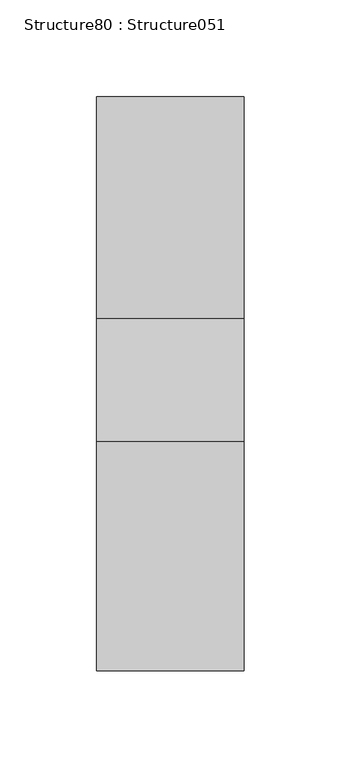
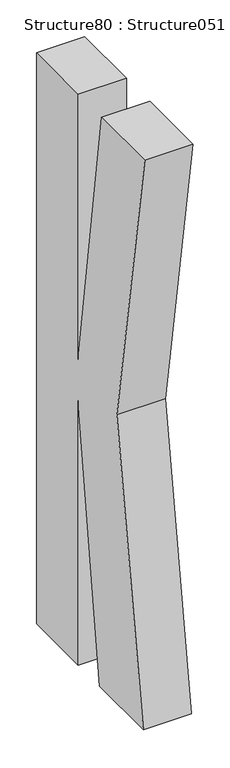
"""IFC4 building model written with IfcOpenShell, lengths in millimetres: proxy geometry, Structure80 : Structure051."""

import ifcopenshell
import ifcopenshell.guid

model = None  # the IFC model being written
_history = None  # IfcOwnerHistory: only IFC2X3 demands one
_inside = {}  # id of a spatial element -> (the spatial element, [elements in it])
_under = {}  # id of a project, library or spatial element -> (it, [spatial elements below it])
_declared = {}  # id of a project -> (the project, [libraries it declares])
_typed = {}  # id of a type object -> (the type object, [elements of that type])
_made_of = {}  # id of a material, layer set ... -> (it, [elements and type objects made of it])


def new_model(schema):
    """Start an empty IFC model of exactly this schema.

    Asked for "IFC4X3", IfcOpenShell would pick the latest addendum, in which some entities
    have other attributes; the version numbers below select the first issue.
    IFC2X3 requires an IfcOwnerHistory on every rooted entity: one is made here for all.
    """
    global model, _history
    if schema == "IFC4X3":
        model = ifcopenshell.file(schema_version=(4, 3, 0, 0))
    else:
        model = ifcopenshell.file(schema=schema)
    _inside.clear()
    _under.clear()
    _declared.clear()
    _typed.clear()
    _made_of.clear()
    _history = None
    if model.schema == "IFC2X3":
        org = make("IfcOrganization", Name="unknown")
        user = make(
            "IfcPersonAndOrganization",
            ThePerson=make("IfcPerson", FamilyName="unknown"),
            TheOrganization=org,
        )
        app = make(
            "IfcApplication",
            ApplicationDeveloper=org,
            Version="unknown",
            ApplicationFullName="unknown",
            ApplicationIdentifier="unknown",
        )
        _history = make(
            "IfcOwnerHistory",
            OwningUser=user,
            OwningApplication=app,
            ChangeAction="ADDED",
            CreationDate=0,
        )
    return model


def make(cls, **values):
    """One entity of the class cls with the attributes given. An attribute that is None is left unset."""
    return model.create_entity(
        cls, **{name: value for name, value in values.items() if value is not None}
    )


def rooted(cls, **values):
    """An entity with a GlobalId (a new one), such as an element, a storey or a relation."""
    return make(cls, GlobalId=ifcopenshell.guid.new(), OwnerHistory=_history, **values)


def si_unit(unit_type, name, prefix=None):
    """IfcSIUnit, for example si_unit("LENGTHUNIT", "METRE", prefix="MILLI")."""
    return make("IfcSIUnit", UnitType=unit_type, Prefix=prefix, Name=name)


def assignment(units):
    """IfcUnitAssignment: the units of a project."""
    return None if units is None else make("IfcUnitAssignment", Units=units)


def point(xyz):
    """IfcCartesianPoint."""
    return None if xyz is None else make("IfcCartesianPoint", Coordinates=xyz)


def direction(xyz):
    """IfcDirection."""
    return None if xyz is None else make("IfcDirection", DirectionRatios=xyz)


def frame(location, z_axis=None, x_axis=None):
    """IfcAxis2Placement3D, a coordinate frame: its origin and axes. An axis left out is left unset."""
    return make(
        "IfcAxis2Placement3D",
        Location=point(location),
        Axis=direction(z_axis),
        RefDirection=direction(x_axis),
    )


def origin():
    """The frame at (0, 0, 0) with its axes left unset."""
    return frame((0.0, 0.0, 0.0))


def place(relative_to, where):
    """IfcLocalPlacement: puts the frame where relative to a parent placement (None: the world)."""
    return make(
        "IfcLocalPlacement", PlacementRelTo=relative_to, RelativePlacement=where
    )


def context(
    kind, dimensions, precision=None, world=None, true_north=None, identifier=None
):
    """IfcGeometricRepresentationContext, for example the 3D "Model" context."""
    return make(
        "IfcGeometricRepresentationContext",
        ContextIdentifier=identifier,
        ContextType=kind,
        CoordinateSpaceDimension=dimensions,
        Precision=precision,
        WorldCoordinateSystem=world,
        TrueNorth=true_north,
    )


def project(units=None, contexts=None):
    """IfcProject with its units and contexts."""
    return rooted(
        "IfcProject",
        Name="project",
        RepresentationContexts=contexts,
        UnitsInContext=assignment(units),
    )


def spatial(cls, under=None, at=None, **own):
    """A site, building, storey or space (cls), placed at a placement, below another one or the project."""
    s = rooted(cls, ObjectPlacement=at, **own)
    if under is not None:
        _under.setdefault(under.id(), (under, []))[1].append(s)
    return s


def polyline(points):
    """IfcPolyline through the points."""
    return make("IfcPolyline", Points=[point(p) for p in points])


def outline(outer, holes=None, kind="AREA"):
    """IfcArbitraryClosedProfileDef: a profile drawn as a closed curve; with holes, ...WithVoids."""
    if holes is None:
        return make("IfcArbitraryClosedProfileDef", ProfileType=kind, OuterCurve=outer)
    return make(
        "IfcArbitraryProfileDefWithVoids",
        ProfileType=kind,
        OuterCurve=outer,
        InnerCurves=holes,
    )


def extrude(swept, where, along, depth):
    """IfcExtrudedAreaSolid: the profile swept, set in the frame where, extruded along a direction by depth."""
    return make(
        "IfcExtrudedAreaSolid",
        SweptArea=swept,
        Position=where,
        ExtrudedDirection=direction(along),
        Depth=depth,
    )


def shape(context_of_items, identifier, shape_type, items):
    """IfcShapeRepresentation: the items that make up one representation, for example the "Body"."""
    return make(
        "IfcShapeRepresentation",
        ContextOfItems=context_of_items,
        RepresentationIdentifier=identifier,
        RepresentationType=shape_type,
        Items=items,
    )


def source(mapping_origin, context_of_items, identifier, shape_type, items):
    """IfcRepresentationMap: a shape defined once, which mapped items show again and again."""
    return make(
        "IfcRepresentationMap",
        MappingOrigin=mapping_origin,
        MappedRepresentation=shape(context_of_items, identifier, shape_type, items),
    )


def transform(
    local_origin,
    x_axis=None,
    y_axis=None,
    z_axis=None,
    scale=None,
    scale2=None,
    scale3=None,
    uniform=True,
):
    """IfcCartesianTransformationOperator3D, or its non-uniform kind. x_axis, y_axis, z_axis: its Axis1, 2, 3."""
    if uniform:
        return make(
            "IfcCartesianTransformationOperator3D",
            Axis1=direction(x_axis),
            Axis2=direction(y_axis),
            LocalOrigin=point(local_origin),
            Scale=scale,
            Axis3=direction(z_axis),
        )
    return make(
        "IfcCartesianTransformationOperator3DnonUniform",
        Axis1=direction(x_axis),
        Axis2=direction(y_axis),
        LocalOrigin=point(local_origin),
        Scale=scale,
        Axis3=direction(z_axis),
        Scale2=scale2,
        Scale3=scale3,
    )


def mapped(mapping_source, mapping_target):
    """IfcMappedItem: shows the shape of a source again, moved by a transform."""
    return make(
        "IfcMappedItem", MappingSource=mapping_source, MappingTarget=mapping_target
    )


def made_of(thing, what):
    """Note that an element or type object is made of a material, layer set ...; save() writes the relation."""
    if what is not None:
        _made_of.setdefault(what.id(), (what, []))[1].append(thing)
    return thing


def element(
    cls,
    number,
    at=None,
    inside=None,
    cuts=None,
    type_object=None,
    material=None,
    context=None,
    identifier="Body",
    shape_type=None,
    held_by="IfcProductDefinitionShape",
    body=None,
    shapes=None,
    **own,
):
    """One element of the class cls, such as IfcWall. Its Tag is "e" and its number.

    at: its placement. inside: the storey or other place that contains it. cuts: it is an
    opening in that element (IfcRelVoidsElement). A single representation is given by context,
    identifier, shape_type and body (its items); several are given by shapes. held_by: the class
    of the entity that holds the representations. save() writes the other relations.
    """
    e = rooted(cls, Tag="e%d" % number, ObjectPlacement=at, **own)
    if body is not None:
        shapes = [shape(context, identifier, shape_type, body)]
    if shapes is not None:
        e.Representation = make(held_by, Representations=shapes)
    if inside is not None:
        _inside.setdefault(inside.id(), (inside, []))[1].append(e)
    if cuts is not None:
        rooted(
            "IfcRelVoidsElement", RelatingBuildingElement=cuts, RelatedOpeningElement=e
        )
    if type_object is not None:
        _typed.setdefault(type_object.id(), (type_object, []))[1].append(e)
    return made_of(e, material)


def aggregate(whole, parts):
    """IfcRelAggregates: a whole, such as a stair, and the parts it consists of."""
    return rooted("IfcRelAggregates", RelatingObject=whole, RelatedObjects=parts)


def save(model, path):
    """Write the relations noted so far, then the file.

    IfcRelAggregates (storeys below a building ...), IfcRelContainedInSpatialStructure (elements
    in a storey), IfcRelDefinesByType, IfcRelAssociatesMaterial and IfcRelDeclares: one each for
    every whole, place, type object, material and project.
    """
    for whole, parts in _under.values():
        aggregate(whole, parts)
    for where, things in _inside.values():
        rooted(
            "IfcRelContainedInSpatialStructure",
            RelatedElements=things,
            RelatingStructure=where,
        )
    for kind, things in _typed.values():
        rooted("IfcRelDefinesByType", RelatedObjects=things, RelatingType=kind)
    for what, things in _made_of.values():
        rooted("IfcRelAssociatesMaterial", RelatedObjects=things, RelatingMaterial=what)
    for by, libraries in _declared.values():
        rooted("IfcRelDeclares", RelatingContext=by, RelatedDefinitions=libraries)
    model.write(path)


def structure80_structure051_452593a8(model_context):
    return source(origin(), model_context, "Body", "SweptSolid", [
        extrude(outline(polyline([(283220.0273561, 3528.5825142), (283292.1031415, 4009.9589531), (283215.9425682, 4480.4419946), (283334.2458585, 4480.4419946), (283398.1520682, 4038.5077532), (283398.1520682, 4480.4419946), (283512.3963918, 4480.4419946), (283512.3963918, 3528.5825142), (283398.1520682, 3528.5825142), (283398.1520682, 3969.1658661), (283339.6865742, 3528.5825142), (283220.0273561, 3528.5825142)])), frame((-59031.6926606, 0.0, 0.0), z_axis=(1.0, 0.0, 0.0), x_axis=(0.0, 1.0, 0.0)), (0.0, 0.0, 1.0), 76.2),
    ])


if __name__ == "__main__":
    model = new_model("IFC4")
    model_context = context("Model", 3, world=origin())
    ifc_project = project(units=[si_unit("LENGTHUNIT", "METRE", prefix="MILLI")], contexts=[model_context])
    site = spatial("IfcSite", under=ifc_project)
    building = spatial("IfcBuilding", under=site)
    placement = place(None, origin())
    structure80_structure051_shape = structure80_structure051_452593a8(model_context)
    element("IfcBuildingElementProxy", 1, Name="Structure80 : Structure051", ObjectType="Structure80 : Structure051", at=placement, inside=building, context=model_context, shape_type="MappedRepresentation", body=[
        mapped(structure80_structure051_shape, transform((0.0, 0.0, 0.0), x_axis=(1.0, 0.0, 0.0), y_axis=(0.0, 1.0, 0.0), z_axis=(0.0, 0.0, 1.0))),
    ])
    save(model, "model.ifc")

# Revit data of these elements
# Type "Structure80 : Structure051"
#   NameOverride = "Structure051"
# Element 1 (IfcBuildingElementProxy, "Structure80 : Structure051")
#   Materials on its faces: "BRUSHED ALUM. LETTERING"
# Materials
#   "BRUSHED ALUM. LETTERING": class "Unassigned", colour RGB 169 181 186, transparency 0, Cost = 0
